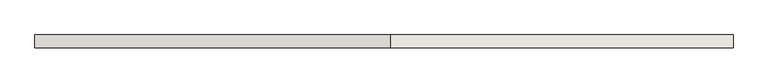
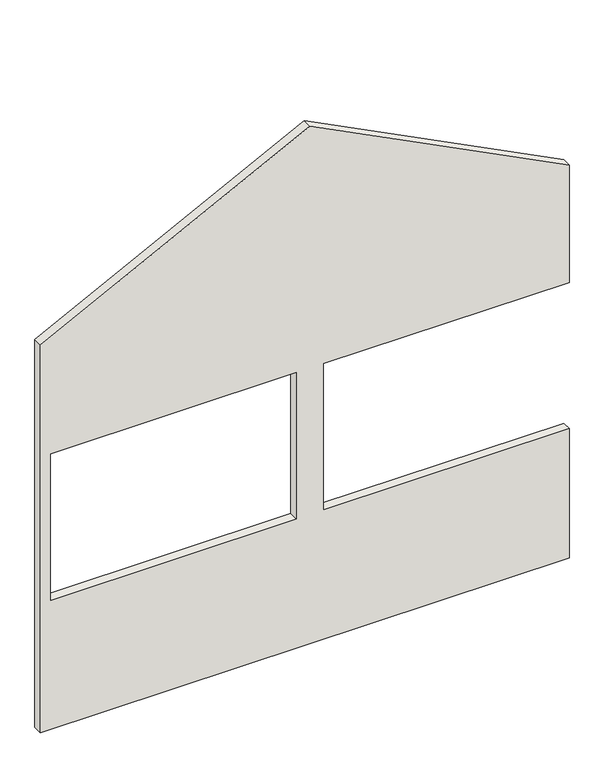
"""IFC4 building model written with IfcOpenShell, lengths in millimetres: wall geometry, 0_3d."""

from ifc_helpers import new_model, si_unit, frame, origin, place, context, project, spatial, polyline, outline, extrude, source, transform, mapped, element, save


def wall_2048f1de(model_context):
    return source(origin(), model_context, "Body", "SweptSolid", [
        extrude(outline(polyline([(1000.0, 3875.0), (1000.0, 2075.0), (2135.0, 2075.0), (2135.0, 3875.0), (3043.5797924, 3875.0), (4011.6781465, 1975.0), (3005.3653837, 0.0), (0.0, 0.0), (0.0, 3875.0), (1000.0, 3875.0)]), holes=[polyline([(2135.0, 1875.0), (1000.0, 1875.0), (1000.0, 75.0), (2135.0, 75.0), (2135.0, 1875.0)])]), frame((0.0, 0.0, 0.0), z_axis=(0.0, 1.0, 0.0), x_axis=(0.0, 0.0, 1.0)), (0.0, 0.0, 1.0), 70.0),
    ])


if __name__ == "__main__":
    model = new_model("IFC4")
    model_context = context("Model", 3, world=origin())
    ifc_project = project(units=[si_unit("LENGTHUNIT", "METRE", prefix="MILLI")], contexts=[model_context])
    site = spatial("IfcSite", under=ifc_project)
    building = spatial("IfcBuilding", under=site)
    placement = place(None, origin())
    wall_shape = wall_2048f1de(model_context)
    element("IfcWall", 1, ObjectType="0_3d", at=placement, inside=building, context=model_context, shape_type="MappedRepresentation", body=[
        mapped(wall_shape, transform((0.0, 0.0, 0.0), x_axis=(1.0, 0.0, 0.0), y_axis=(0.0, 1.0, 0.0), z_axis=(0.0, 0.0, 1.0))),
    ])
    save(model, "model.ifc")

# Revit data of these elements
# Element 1 (IfcWall, "0_3d")
#   Materials on its faces: "Glass_Simple"
# Materials
#   "Glass_Simple": class "Unassigned", colour RGB 255 255 255, transparency 0.9
